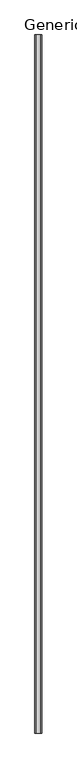
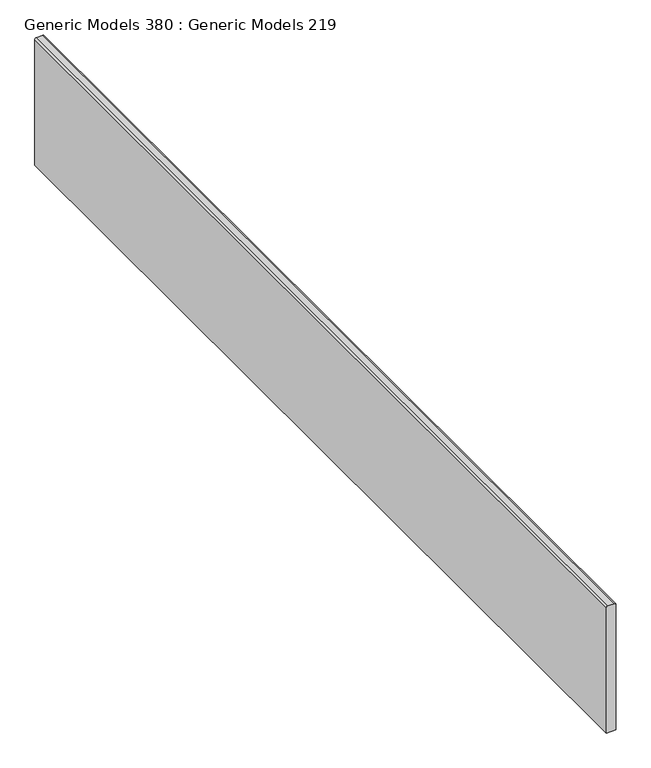
"""IFC4 building model written with IfcOpenShell, lengths in millimetres: proxy geometry, Generic Models 380 : Generic Models 219."""

from ifc_helpers import new_model, si_unit, point, frame, frame_2d, origin, place, context, project, spatial, polyline, circle_curve, trimmed, segment, composite_curve, outline, extrude, source, transform, mapped, element, save


def generic_models_380_generic_models_219_5e198b85(model_context):
    return source(origin(), model_context, "Body", "SweptSolid", [
        extrude(outline(composite_curve([segment(trimmed(circle_curve(frame_2d((128953.0568, -6860.8508813)), 8.8392), [point((128953.0568, -6852.0116813))], [point((128961.896, -6860.8508813))], False, "CARTESIAN"), True, "CONTINUOUS"), segment(polyline([(128961.896, -6860.8508813), (128961.896, -6893.9724813)]), True, "CONTINUOUS"), segment(trimmed(circle_curve(frame_2d((128953.0568, -6893.9724813)), 8.8392), [point((128961.896, -6893.9724813))], [point((128953.0568, -6902.8116813))], False, "CARTESIAN"), True, "CONTINUOUS"), segment(polyline([(128953.0568, -6902.8116813), (128256.931023, -6902.8116813), (128256.931023, -6852.0116813), (128953.0568, -6852.0116813)]), True, "CONTINUOUS")], self_intersect=False)), frame((0.0, -7154.7506628, 0.0), z_axis=(0.0, 1.0, 0.0), x_axis=(0.0, 0.0, 1.0)), (0.0, 0.0, 1.0), 5204.497286),
    ])


if __name__ == "__main__":
    model = new_model("IFC4")
    model_context = context("Model", 3, world=origin())
    ifc_project = project(units=[si_unit("LENGTHUNIT", "METRE", prefix="MILLI")], contexts=[model_context])
    site = spatial("IfcSite", under=ifc_project)
    building = spatial("IfcBuilding", under=site)
    placement = place(None, origin())
    generic_models_380_generic_models_219_shape = generic_models_380_generic_models_219_5e198b85(model_context)
    element("IfcBuildingElementProxy", 1, Name="Generic Models 380 : Generic Models 219", ObjectType="Generic Models 380 : Generic Models 219", at=placement, inside=building, context=model_context, shape_type="MappedRepresentation", body=[
        mapped(generic_models_380_generic_models_219_shape, transform((0.0, 0.0, 0.0), x_axis=(1.0, 0.0, 0.0), y_axis=(0.0, 1.0, 0.0), z_axis=(0.0, 0.0, 1.0))),
    ])
    save(model, "model.ifc")

# Revit data of these elements
# Element 1 (IfcBuildingElementProxy, "Generic Models 380 : Generic Models 219")
#   Materials on its faces: "_PLANTATION STYLE SHUTTERS BY OWNER"
# Materials
#   "_PLANTATION STYLE SHUTTERS BY OWNER": class "Metal", colour RGB 209 202 188, transparency 0, Description = "Structural steel 50ksi", Cost = 0
